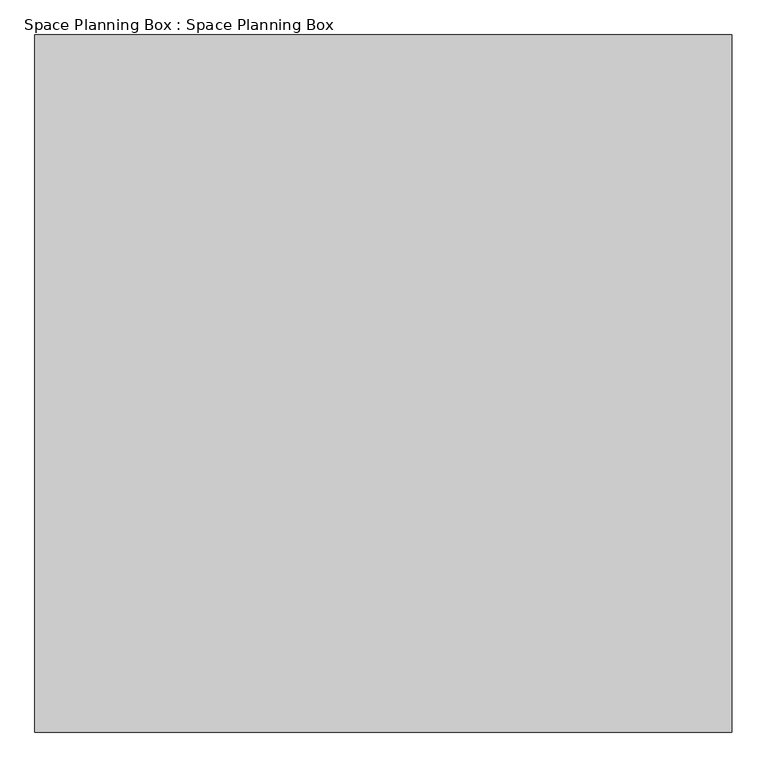
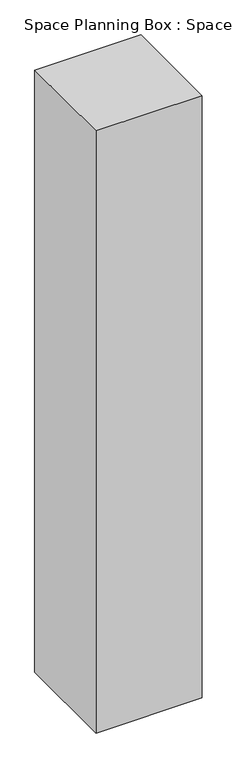
"""IFC4 building model written with IfcOpenShell, lengths in millimetres: proxy geometry, Space Planning Box : Space Planning Box."""

from ifc_helpers import new_model, si_unit, origin, origin_with_axes, place, context, project, spatial, polyline, outline, extrude, source, transform, mapped, element, save


def space_planning_box_space_planning_box_ed4b717c(model_context):
    return source(origin(), model_context, "Body", "SweptSolid", [
        extrude(outline(polyline([(500.0, 500.0), (500.0, -500.0), (-500.0, -500.0), (-500.0, 500.0), (500.0, 500.0)])), origin_with_axes(), (0.0, 0.0, 1.0), 6000.0),
    ])


if __name__ == "__main__":
    model = new_model("IFC4")
    model_context = context("Model", 3, world=origin())
    ifc_project = project(units=[si_unit("LENGTHUNIT", "METRE", prefix="MILLI")], contexts=[model_context])
    site = spatial("IfcSite", under=ifc_project)
    building = spatial("IfcBuilding", under=site)
    placement = place(None, origin())
    space_planning_box_space_planning_box_shape = space_planning_box_space_planning_box_ed4b717c(model_context)
    element("IfcBuildingElementProxy", 1, Name="Space Planning Box : Space Planning Box", ObjectType="Space Planning Box : Space Planning Box", at=placement, inside=building, context=model_context, shape_type="MappedRepresentation", body=[
        mapped(space_planning_box_space_planning_box_shape, transform((0.0, 0.0, 0.0), x_axis=(1.0, 0.0, 0.0), y_axis=(0.0, 1.0, 0.0), z_axis=(0.0, 0.0, 1.0))),
    ])
    save(model, "model.ifc")

# Revit data of these elements
# Type "Space Planning Box : Space Planning Box"
#   Type Comments = "..."
#   Room Name [instance default] = "?"
#   Assembly Code = "..."
#   Width [instance default] = 1524 mm
#   Program Area [instance default] = 0 m²
#   Length [instance default] = 1524 mm
#   Height [instance default] = 1524 mm
#   Area [instance default] = 2.32258 m²
#   Fill Color [instance default] = Cyan
#   Default Elevation = 0
# Element 1 (IfcBuildingElementProxy, "Space Planning Box : Space Planning Box")
#   Room Name = "Fire Gas Room"
#   Width = 1000 mm
#   Length = 1000 mm
#   Height = 6000 mm
#   Area = 1 m²
#   Materials on its faces: "Cyan"
# Materials
#   "Cyan": class "Generic", colour RGB 0 255 255, transparency 0.2, Cost = 0
